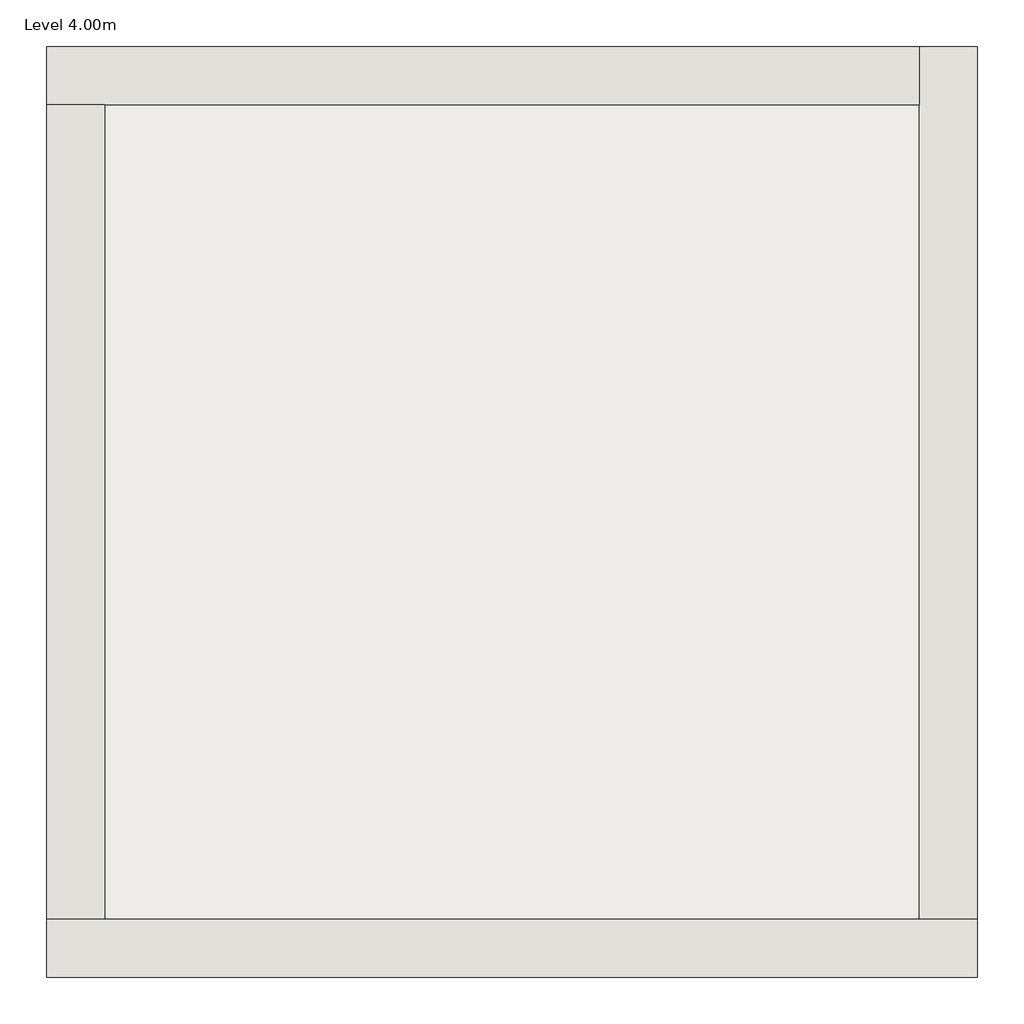
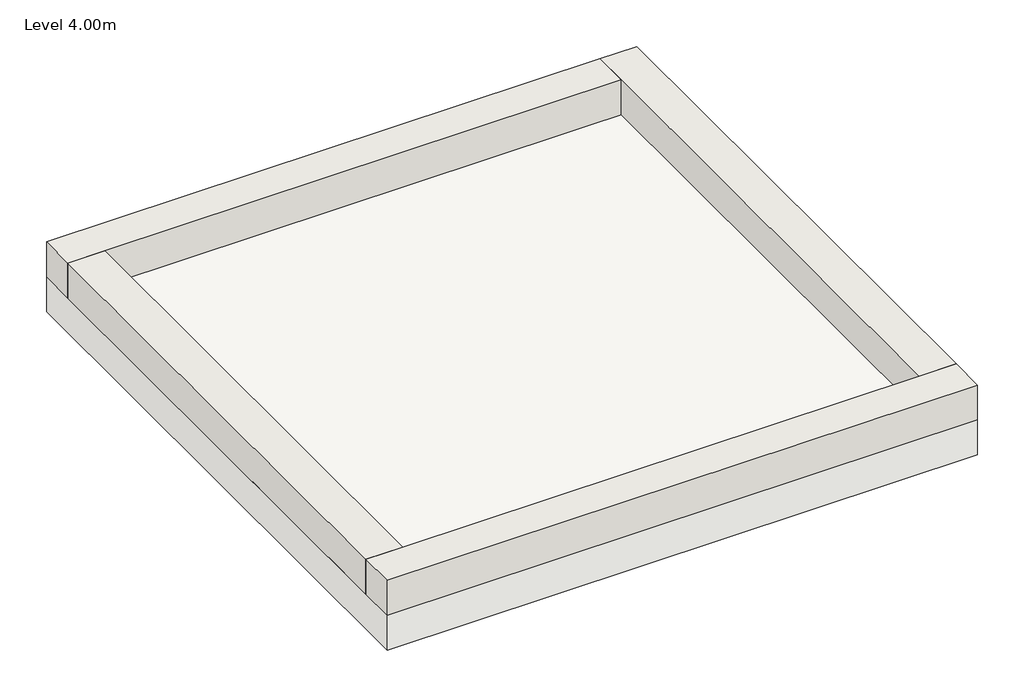
# One storey: 4 walls, 1 slab.
"""IFC4 building model written with IfcOpenShell, lengths in millimetres."""

from ifc_helpers import new_model, si_unit, frame, origin, place, context, project, spatial, polyline, outline, extrude, faceted_brep, element, save

model = new_model("IFC4")

# Units and contexts
model_context = context("Model", 3, world=origin())
ifc_project = project(units=[si_unit("LENGTHUNIT", "METRE", prefix="MILLI")], contexts=[model_context])

# Site, building, storey
site = spatial("IfcSite", under=ifc_project)
building = spatial("IfcBuilding", under=site)
storey = spatial("IfcBuildingStorey", under=building, Name="Level 4.00m", Elevation=4000.0)

# Slab
placement = place(None, origin())
element("IfcSlab", 1, ObjectType="FOR INT AC-NH", at=placement, inside=storey, context=model_context, shape_type="SweptSolid", body=[
    extrude(outline(polyline([(7999.99416, 0.0), (0.0, 0.0), (0.0, 7999.99416), (7999.99416, 7999.99416), (7999.99416, 0.0)])), frame((0.0, 0.0, 3500.0000028), z_axis=(0.0, 0.0, 1.0), x_axis=(1.0, 0.0, 0.0)), (0.0, 0.0, 1.0), 499.9999972),
])

# Walls
element("IfcWall", 2, ObjectType="MURO EXTERIOR0.60", at=placement, inside=storey, context=model_context, shape_type="Brep", body=[
    faceted_brep([(0.0, 0.0, 4000.0), (7999.99416, 0.0, 4000.0), (7999.99416, 0.0, 4499.99392), (0.0, 0.0, 4499.99392), (0.0, 500.000016, 4000.0), (0.0, 500.000016, 4499.99392), (500.000016, 500.000016, 4499.99392), (7499.994144, 500.000016, 4499.99392), (7999.99416, 500.000016, 4499.99392), (7999.99416, 500.000016, 4000.0), (7499.994144, 500.000016, 4000.0), (500.000016, 500.000016, 4000.0)], [[[0, 1, 2, 3]], [[4, 5, 6, 7, 8, 9, 10, 11]], [[1, 0, 4, 11, 10, 9]], [[3, 2, 8, 7, 6, 5]], [[2, 1, 9, 8]], [[0, 3, 5, 4]]]),
])
element("IfcWall", 3, ObjectType="MURO EXTERIOR0.60", at=placement, inside=storey, context=model_context, shape_type="Brep", body=[
    faceted_brep([(7999.99416, 500.000016, 4000.0), (7999.99416, 7999.99416, 4000.0), (7999.99416, 7999.99416, 4499.99392), (7999.99416, 500.000016, 4499.99392), (7499.994144, 500.000016, 4000.0), (7499.994144, 500.000016, 4499.99392), (7499.994144, 7499.994144, 4499.99392), (7499.994144, 7999.99416, 4499.99392), (7499.994144, 7999.99416, 4000.0), (7499.994144, 7499.994144, 4000.0)], [[[0, 1, 2, 3]], [[4, 5, 6, 7, 8, 9]], [[1, 0, 4, 9, 8]], [[3, 2, 7, 6, 5]], [[2, 1, 8, 7]], [[0, 3, 5, 4]]]),
])
element("IfcWall", 4, ObjectType="MURO EXTERIOR0.60", at=placement, inside=storey, context=model_context, shape_type="Brep", body=[
    faceted_brep([(7499.994144, 7999.99416, 4000.0), (0.0, 7999.99416, 4000.0), (0.0, 7999.99416, 4499.99392), (7499.994144, 7999.99416, 4499.99392), (7499.994144, 7499.994144, 4000.0), (7499.994144, 7499.994144, 4499.99392), (500.000016, 7499.994144, 4499.99392), (0.0, 7499.994144, 4499.99392), (0.0, 7499.994144, 4000.0), (500.000016, 7499.994144, 4000.0)], [[[0, 1, 2, 3]], [[4, 5, 6, 7, 8, 9]], [[1, 0, 4, 9, 8]], [[3, 2, 7, 6, 5]], [[2, 1, 8, 7]], [[0, 3, 5, 4]]]),
])
element("IfcWall", 5, ObjectType="MURO EXTERIOR0.60", at=placement, inside=storey, context=model_context, shape_type="SweptSolid", body=[
    extrude(outline(polyline([(0.0, 500.000016), (0.0, 7499.994144), (500.000016, 7499.994144), (500.000016, 500.000016), (0.0, 500.000016)])), frame((0.0, 0.0, 4000.0), z_axis=(0.0, 0.0, 1.0), x_axis=(1.0, 0.0, 0.0)), (0.0, 0.0, 1.0), 499.99392),
])

save(model, "model.ifc")

# Revit data of these elements
# Type "FOR INT AC-NH"
#   Layers, outside or top first: 0.010 m "Plaqueta o baldosa de gres" (function 1); 0.055 m "Mortero de cemento o cal para albañilería y para revoco-enlucido d entre 1000 y 1250" (function 1); 0.120 m "Poliestireno Expandido XPS" (function 1); 0.250 m "FU Entrevigado cerámico -Canto 250 mm" (function 1); 0.050 m "Cámara de aire sin ventilar horizontal 5 cm" (function 1); 0.015 m "Placa de yeso laminado (PYL) d entre 750 y 900" (function 1)
# Type "MURO EXTERIOR0.60"
#   Description = "Metal Studs with Brick over sheathing on exterior and Gypsum Wall Board (GWB) on interior, Exterior Function"
#   Assembly Code = "B2010158"
#   Type Mark = "W10"
#   Layers, outside or top first: 0.030 m no material (function 1); 0.140 m no material (function 1); 0.240 m no material (function 1); 0.010 m no material (function 1); 0.050 m no material (function 1); 0.015 m no material (function 1); 0.015 m no material (function 1)
# Element 1 (IfcSlab, "FOR INT AC-NH")
#   Height Offset From Level = 0.000 m
#   Phase Created = New Construction
#   Materials on its faces: "Placa de yeso laminado (PYL) d entre 750 y 900", "Plaqueta o baldosa de gres"
# Elements 2, 3, 4, 5 (IfcWall, "MURO EXTERIOR0.60")
#   Top Offset = 0.000 m
#   Base Offset = 0.000 m
#   Unconnected Height = 0.499994 m
#   wall height = 0.499994 m
#   Phase Created = New Construction
#   Base Constraint = Level 4.00m
#   Materials on its faces: "Default Wall"
# Materials
#   "Plaqueta o baldosa de gres": class "Cerámicos", colour RGB 0 0 0, transparency 0, Comments = "CTE"
#   "Mortero de cemento o cal para albañilería y para revoco-enlucido d entre 1000 y 1250": class "Morteros", colour RGB 0 0 0, transparency 0, Comments = "CTE"
#   "Poliestireno Expandido XPS": class "Plásticos", colour RGB 0 0 0, transparency 0, Comments = "CTE"
#   "FU Entrevigado cerámico -Canto 250 mm": class "Forjados unidireccionales", colour RGB 0 0 0, transparency 0, Comments = "CTE"
#   "Cámara de aire sin ventilar horizontal 5 cm": class "Cámaras de aire", colour RGB 0 0 0, transparency 0, Comments = "CTE"
#   "Placa de yeso laminado (PYL) d entre 750 y 900": class "Yesos", colour RGB 0 0 0, transparency 0, Comments = "CTE"
#   "Default Wall": class "Miscellaneous", colour RGB 192 192 192, transparency 0, Cost = 0
